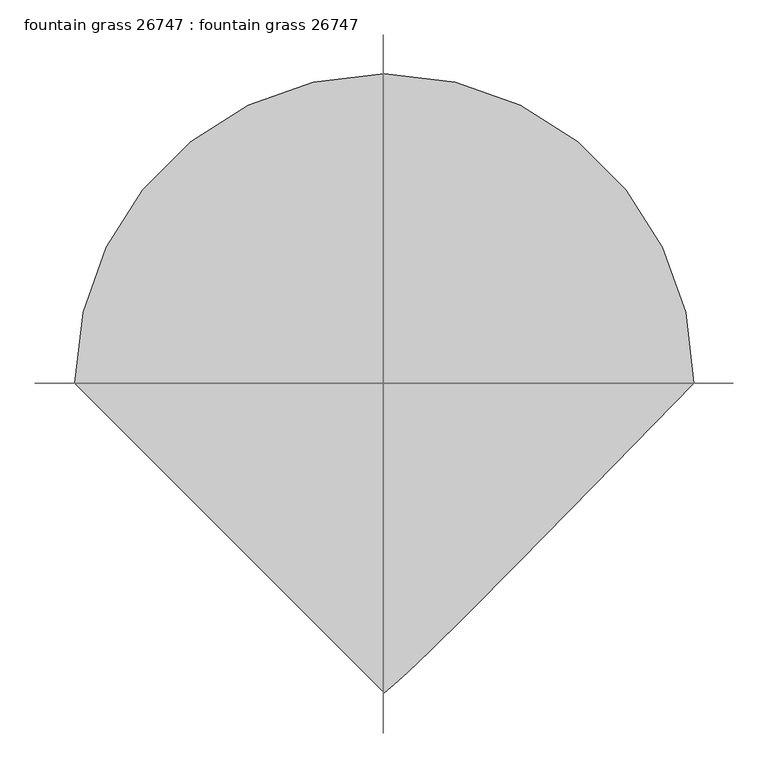
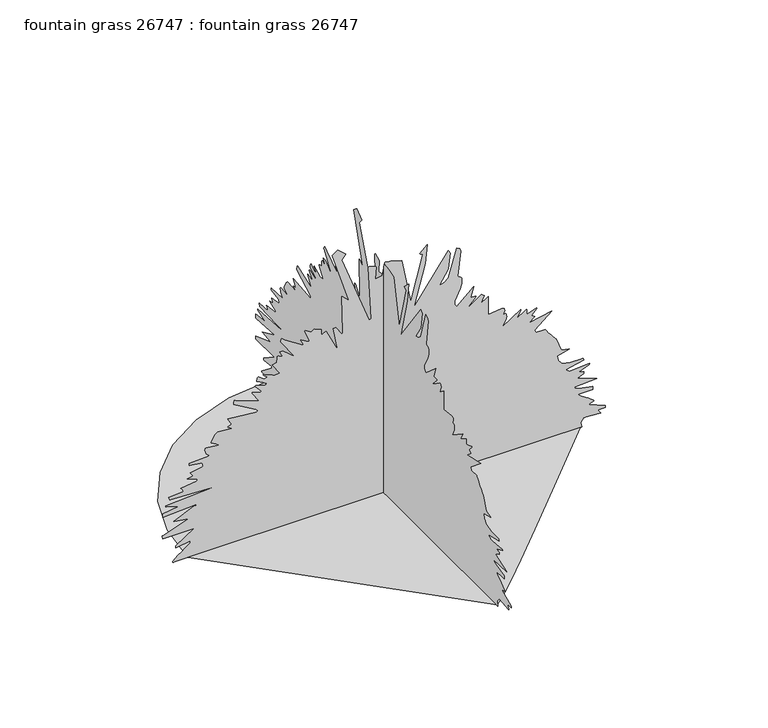
"""IFC4 building model written with IfcOpenShell, lengths in millimetres: proxy geometry, fountain grass 26747 : fountain grass 26747."""

from ifc_helpers import new_model, si_unit, origin, place, context, project, spatial, triangles, source, transform, mapped, element, save


def fountain_grass_26747_fountain_grass_26747_29f4d5b1(model_context):
    return source(origin(), model_context, "Body", "Tessellation", [
        triangles([(-987.0455658, 0.0, 0.0001807), (-960.952173, 226.1654466, 0.0001807), (-886.6343983, 433.862035, 0.0001807), (-770.0484913, 617.1406734, 0.0001807), (-617.1406734, 770.0484913, 0.0001807), (-433.862035, 886.6343983, 0.0001807), (-226.1654466, 960.952173, 0.0001807), (4.31e-05, 987.0455658, 0.0001807), (226.1657009, 960.952173, 0.0001807), (433.862035, 886.6343983, 0.0001807), (617.1406734, 770.0484913, 0.0001807), (770.0484913, 617.1406734, 0.0001807), (886.6343983, 433.862035, 0.0001807), (960.952173, 226.1654466, 0.0001807), (987.0455658, -8.63e-05, 0.0001807), (666.2769184, -329.0287173, 0.0001807), (428.4772619, -571.2784656, 0.0001807), (259.8137924, -741.2118793, 0.0001807), (146.4631077, -853.2918114, 0.0001807), (74.5956602, -921.9810053, 0.0001807), (30.3837036, -961.7446392, 0.0001807), (-0.0001294, -987.0455658, 0.0001807), (-192.732222, 8.8e-06, 1335.7745705), (-213.2038286, 7.2e-06, 1310.1839813), (-75.0206025, -1.47e-05, 941.6939009), (-74.0421966, -1.47e-05, 941.9784039), (-72.5994794, -1.47e-05, 942.7098999), (-70.8743122, -1.46e-05, 943.7080948), (-69.0480519, -1.45e-05, 944.7977812), (-67.3038361, -1.45e-05, 945.7985195), (-65.8220043, -1.44e-05, 946.5300882), (-64.7846675, -1.44e-05, 946.8119751), (-80.1384406, 2.1e-06, 1223.1789722), (-79.3512975, 2.1e-06, 1223.3695129), (-78.4244554, 2.1e-06, 1223.8850338), (-77.4526488, 2.1e-06, 1224.6394936), (-76.5311389, 2.2e-06, 1225.5436535), (-75.2199908, 2.3e-06, 1227.4587982), (-75.0206025, 2.4e-06, 1228.2971191), (-39.1952093, 1.4e-06, 1212.9427511), (-44.3130519, -2.2e-06, 1151.5281858), (-8.4877319, -1.9e-06, 1156.6462601), (4.7327266, 1.8e-06, 1221.0427654), (6.8660195, 2.1e-06, 1223.1789722), (43.5436857, 1.6e-06, 1215.9958351), (88.7523407, 8e-07, 1202.7066027), (134.8136643, -1.32e-05, 967.2843447), (196.2285203, 5e-07, 1197.5909992), (183.550624, 1e-06, 1203.2526449), (181.3428736, 1.1e-06, 1205.4269308), (180.8747518, 1.1e-06, 1207.8246769), (216.700145, 3.3e-06, 1243.6512691), (206.4644507, -2.5e-06, 1146.4100389), (150.1674419, -1.53e-05, 931.4576797), (324.1773419, 3.2e-06, 1172.2011972), (334.4109833, 2.3e-06, 1156.8469019), (324.1773419, -2.6e-06, 1074.959967), (278.1144741, -6.8e-06, 1003.3091806), (303.186799, -6.4e-06, 1010.2737991), (322.3333048, -5.3e-06, 1028.8183794), (365.1195376, 3.2e-06, 1172.2011972), (380.7405318, 2.8e-06, 1165.3635332), (386.8136713, 1.8e-06, 1149.1050053), (371.0377447, -5.8e-06, 1020.4236883), (372.5033166, -6e-06, 1017.0835579), (375.3150999, -6.2e-06, 1014.6375589), (378.9295232, -6.3e-06, 1012.7299719), (382.8157322, -6.4e-06, 1011.0028244), (386.4301191, -6.5e-06, 1009.0952374), (389.2419024, -6.6e-06, 1006.6492384), (390.7100178, -6.8e-06, 1003.3091806), (390.8116467, -8.5e-06, 974.9780611), (383.7479064, -1e-05, 950.4898756), (355.0433722, -1.34e-05, 892.7557543), (354.7944775, -1.44e-05, 876.299128), (365.1195376, -1.54e-05, 860.0101513), (452.1246194, -1.08e-05, 936.7764685), (436.7703604, -1.39e-05, 885.5980516), (437.4358357, -1.38e-05, 884.2035873), (460.8495229, -1.41e-05, 882.1284233), (462.3608042, -1.42e-05, 880.4799774), (460.8800079, -1.46e-05, 876.8274387), (425.4318083, -1.61e-05, 841.6561117), (426.5341393, -1.66e-05, 839.537709), (430.7911832, -1.6e-05, 840.3353348), (487.9487409, -1.42e-05, 880.4799774), (489.1120783, -1.43e-05, 881.361319), (491.0831062, -1.43e-05, 880.6425402), (503.3030362, -1.48e-05, 870.2437563), (487.9487409, -1.69e-05, 834.4196348), (523.7754058, -1.54e-05, 860.0101513), (523.7754058, -2.12e-05, 762.7688484), (593.7116893, -2.08e-05, 769.8782982), (604.2222033, -2.1e-05, 765.8219324), (607.2778307, -2.16e-05, 755.5679798), (600.5443027, -2.27e-05, 737.1784046), (610.7779804, -2.27e-05, 737.1784046), (611.8422323, -2.27e-05, 736.5230667), (614.1129513, -2.29e-05, 734.0897123), (616.2186367, -2.32e-05, 729.1722799), (616.7773962, -2.37e-05, 721.0722656), (614.4152584, -2.44e-05, 709.086006), (595.4261922, -2.67e-05, 670.6456924), (687.546841, -2.3e-05, 732.0602577), (687.8186268, -2.35e-05, 728.1842588), (667.0770149, -2.55e-05, 691.118062), (716.0887762, -2.38e-05, 722.0933516), (718.2554317, -2.36e-05, 721.8266527), (719.3450455, -2.39e-05, 719.0986942), (717.5061316, -2.5e-05, 697.6534916), (718.2554317, -2.51e-05, 696.2361362), (720.4347319, -2.49e-05, 695.6976517), (766.5382404, -2.45e-05, 712.7029364), (769.4337759, -2.42e-05, 711.5904316), (768.6387663, -2.44e-05, 709.4415802), (744.2522461, -2.59e-05, 683.2440514), (743.8433321, -2.61e-05, 680.8819136), (759.1976274, -2.67e-05, 670.6456924), (728.4915802, -2.82e-05, 645.0577194), (845.0825741, -2.67e-05, 669.6881201), (759.1976274, -3.09e-05, 598.994906), (764.3157017, -3.19e-05, 583.6431541), (810.3760443, -3.19e-05, 583.6431541), (812.6900019, -3.21e-05, 579.4623047), (818.8519804, -3.26e-05, 570.8923699), (827.7013676, -3.33e-05, 559.353176), (838.0696301, -3.41e-05, 546.269636), (848.7985537, -3.49e-05, 533.064192), (858.7223665, -3.56e-05, 521.1643006), (866.6750788, -3.61e-05, 511.9923677), (892.2629791, -4.01e-05, 445.4596919), (933.2077909, -4.07e-05, 435.2234708), (871.793153, -4.16e-05, 419.8692118), (876.9112272, -4.31e-05, 394.2787316), (879.8754358, -4.33e-05, 391.6269676), (882.8904408, -4.35e-05, 388.2919604), (885.7733316, -4.37e-05, 384.6267408), (888.3361839, -4.39e-05, 380.9920063), (890.3960873, -4.41e-05, 377.7407876), (891.7651897, -4.43e-05, 375.2261882), (892.2629791, -4.44e-05, 373.8088692), (895.890156, -4.44e-05, 372.7801892), (938.3258652, -4.5e-05, 363.5726844), (999.7404305, -4.5e-05, 363.5726844), (1000.5278824, -4.5e-05, 362.5440044), (1001.4549334, -4.51e-05, 361.080976), (1002.425223, -4.52e-05, 359.3588428), (1003.3472597, -4.53e-05, 357.5503776), (1004.1219217, -4.54e-05, 355.8282443), (1004.6578629, -4.55e-05, 354.3652159), (1004.8585773, -4.56e-05, 353.3364996), (912.7354214, -4.68e-05, 332.86413), (913.6015022, -4.69e-05, 331.6373154), (915.8976557, -4.7e-05, 329.6383458), (919.1819029, -4.71e-05, 327.1415142), (923.0020912, -4.73e-05, 324.4110123), (926.9110823, -4.75e-05, 321.7160823), (930.4620283, -4.76e-05, 319.3259302), (933.2077909, -4.77e-05, 317.5123781), (949.6695042, -4.77e-05, 318.6757155), (1032.0797356, -4.76e-05, 324.6954789), (1035.5645519, -4.74e-05, 322.6279452), (1033.032221, -4.76e-05, 319.7526484), (979.2680609, -4.89e-05, 297.0400085), (1004.8585773, -4.92e-05, 291.9219162), (1004.8585773, -4.99e-05, 281.6857132), (975.3971489, -5.07e-05, 267.6446189), (974.1499866, -5.08e-05, 266.331436), (1071.3912169, -5.29e-05, 230.5068058), (958.7956913, -5.32e-05, 225.3889678), (958.7956913, -5.35e-05, 220.2708572), (979.2680609, -5.41e-05, 210.0351811), (1050.9188473, -5.5e-05, 194.6814126), (1050.9188473, -5.6e-05, 179.327626), (974.1499866, -5.6e-05, 179.327626), (978.767728, -5.62e-05, 175.5818881), (990.6523224, -5.67e-05, 167.0838239), (1006.8625975, -5.74e-05, 155.6789786), (1024.4520761, -5.81e-05, 143.2134423), (1051.9830992, -5.94e-05, 122.4842661), (1056.0369942, -5.96e-05, 117.9127791), (1055.1428627, -5.97e-05, 116.2480642), (1031.9527084, -6.02e-05, 108.5996212), (1030.4464777, -6.02e-05, 107.6770939), (1112.3334852, -6.24e-05, 71.8517007), (1112.3334852, -6.3e-05, 61.6157658), (1076.5093637, -6.3e-05, 61.6157658), (1088.8461107, -6.4e-05, 43.7974311), (1091.8611156, -6.42e-05, 41.1441501), (1004.8585773, -6.39e-05, 46.2622425), (989.504282, -6.51e-05, 25.7906269), (994.6223562, -6.66e-05, 0.2009925), (-1062.775609, -7.09e-05, 6.89e-05), (-1062.775609, -7.05e-05, 5.1179681), (-1049.4888474, -6.99e-05, 15.7529118), (-1033.944084, -6.92e-05, 27.9602914), (-1017.6728388, -6.84e-05, 40.5703616), (-1002.191589, -6.77e-05, 52.4138656), (-989.0343979, -6.71e-05, 62.3213777), (-979.7176701, -6.67e-05, 69.1234924), (-975.7730707, -6.66e-05, 71.6507864), (-975.7730707, -6.6e-05, 81.8864716), (-1047.4213137, -6.66e-05, 71.6507864), (-1047.4213137, -6.6e-05, 81.8864716), (-955.3006285, -6.23e-05, 143.3013185), (-1113.9564966, -6.23e-05, 143.3013185), (-1114.0479881, -6.22e-05, 144.6553964), (-1114.2638906, -6.21e-05, 147.0447673), (-1114.5102419, -6.19e-05, 150.0158069), (-1114.6931522, -6.17e-05, 153.1156177), (-1114.7261444, -6.16e-05, 155.891066), (-1114.5102419, -6.14e-05, 157.8885276), (-1113.9564966, -6.14e-05, 158.6551051), (-986.0066757, -5.87e-05, 204.7161744), (-1054.7643974, -5.81e-05, 213.3275311), (-1057.6574621, -5.8e-05, 214.9521049), (-955.3006285, -5.53e-05, 261.0126836), (-945.06448, -5.53e-05, 261.0126836), (-945.06448, -5.5e-05, 266.130776), (-1113.9564966, -5.56e-05, 255.8945912), (-1113.9564966, -5.44e-05, 276.3669608), (-1032.0695618, -5.38e-05, 286.6031456), (-1098.6022739, -5.26e-05, 307.0755152), (-1098.6022739, -5.22e-05, 312.1910823), (-852.941324, -5.13e-05, 327.5453776), (-1078.1298317, -5.07e-05, 337.7815624), (-1082.9660191, -4.99e-05, 351.3121319), (-1083.2479786, -4.98e-05, 353.1358578), (-1006.4790453, -4.95e-05, 358.253932), (-1021.1679016, -4.84e-05, 377.3064754), (-1021.8333406, -4.83e-05, 378.7237945), (-939.9464058, -4.77e-05, 388.9599792), (-939.9464058, -4.71e-05, 399.196164), (-983.6648129, -4.62e-05, 414.4208888), (-989.0952953, -4.6e-05, 417.5603411), (-991.1248226, -4.58e-05, 419.6685336), (-960.4187754, -4.55e-05, 424.7866442), (-975.1050156, -4.44e-05, 443.8391513), (-975.7730707, -4.43e-05, 445.2590137), (-909.2403585, -4.37e-05, 455.4926551), (-914.3558893, -4.25e-05, 475.965061), (-980.8911449, -4.19e-05, 486.2012458), (-980.8911449, -4.13e-05, 496.4374306), (-878.5317678, -4.1e-05, 501.5555048), (-879.1134184, -4.09e-05, 503.3716003), (-888.6028828, -4.02e-05, 513.6840159), (-893.8860632, -4e-05, 516.9098001), (-900.7211838, -3.88e-05, 540.5851356), (-900.558621, -3.85e-05, 544.4840255), (-899.0041374, -3.82e-05, 547.6158474), (-894.7090508, -3.84e-05, 548.9721963), (-839.7257063, -3.85e-05, 543.0539892), (-832.4714979, -3.85e-05, 542.4977368), (-834.0945093, -3.85e-05, 545.8555987), (-865.9461262, -3.72e-05, 565.5888419), (-868.2956194, -3.7e-05, 568.088217), (-868.4048424, -3.65e-05, 572.164894), (-848.5039495, -3.46e-05, 604.96896), (-842.4562082, -3.44e-05, 611.1792641), (-837.5895721, -3.42e-05, 614.1485596), (-765.9387857, -3.46e-05, 609.030449), (-780.5183464, -3.41e-05, 617.4352776), (-785.6364206, -3.37e-05, 622.5609821), (-786.4086119, -3.36e-05, 624.384708), (-767.3586119, -3.34e-05, 628.6646067), (-765.9387857, -3.33e-05, 629.5027822), (-786.4086119, -3.12e-05, 665.3269037), (-637.9889648, -3.21e-05, 649.9752245), (-637.7984241, -3.21e-05, 650.9530718), (-637.2828306, -3.2e-05, 652.395789), (-636.5284435, -3.19e-05, 654.1204657), (-635.6242109, -3.18e-05, 655.946735), (-634.6564648, -3.17e-05, 657.6916866), (-633.7090662, -3.16e-05, 659.1725555), (-632.8733614, -3.15e-05, 660.2088295), (-755.7025646, -2.72e-05, 731.8596159), (-755.710195, -2.71e-05, 734.6180958), (-755.6593987, -2.69e-05, 738.1944036), (-755.4384092, -2.67e-05, 742.1339161), (-754.9329895, -2.65e-05, 745.9743793), (-754.0313004, -2.63e-05, 749.26117), (-752.6190319, -2.61e-05, 751.5344324), (-750.5844904, -2.6e-05, 752.3319855), (-627.7552872, -2.88e-05, 706.2717155), (-663.6860882, -2.56e-05, 759.6675116), (-663.5794086, -2.54e-05, 762.5682066), (-660.4755283, -2.56e-05, 763.5054314), (-620.4934484, -2.58e-05, 751.3083561), (-617.5191387, -2.6e-05, 752.3319855), (-618.27854, -2.56e-05, 755.4434961), (-647.6638103, -2.37e-05, 790.1982788), (-648.2251133, -2.36e-05, 793.2742538), (-645.0653498, -2.38e-05, 794.1149729), (-597.0467328, -2.45e-05, 777.9225019), (-596.4675894, -2.44e-05, 778.9130665), (-595.0452198, -2.43e-05, 780.3888485), (-593.2570295, -2.42e-05, 782.1490608), (-591.5755551, -2.41e-05, 784.0032354), (-590.4782747, -2.4e-05, 785.7507305), (-590.4376522, -2.39e-05, 787.201078), (-591.9286222, -2.39e-05, 788.1586504), (-637.9889648, -2.24e-05, 813.7466234), (-639.6145197, -2.21e-05, 815.2045286), (-640.0666723, -2.19e-05, 818.265243), (-638.3851616, -2.15e-05, 826.5253492), (-636.7163681, -2.14e-05, 830.3861601), (-634.8012234, -2.12e-05, 833.1724726), (-632.8733614, -2.11e-05, 834.218993), (-630.4730719, -2.12e-05, 834.2443548), (-602.164807, -2.24e-05, 813.7466234), (-586.810548, -2.2e-05, 818.8646976), (-606.0256179, -2.11e-05, 834.9200403), (-607.7909171, -2.1e-05, 837.6987951), (-607.2829176, -2.08e-05, 839.3370672), (-603.6684943, -2.09e-05, 838.9128925), (-561.8702826, -2.2e-05, 820.0915123), (-550.9864265, -2.24e-05, 813.7466234), (-525.3959464, -2.2e-05, 818.8646976), (-559.8662261, -1.89e-05, 871.7906096), (-561.2226113, -1.87e-05, 875.1611887), (-540.7502054, -1.84e-05, 880.2793356), (-537.9714506, -1.73e-05, 906.7536644), (-536.9859366, -1.7e-05, 909.870262), (-535.6321312, -1.66e-05, 910.9878536), (-533.2191244, -1.68e-05, 912.2654646), (-529.3558064, -1.69e-05, 911.5212513), (-510.0416511, -1.72e-05, 900.7517052), (-525.3959464, -1.53e-05, 931.4576797), (-510.0416511, -1.53e-05, 931.4576797), (-448.6270494, -1.84e-05, 880.2793356), (-520.2778358, -1.23e-05, 982.63864), (-520.4962818, -1.22e-05, 984.7163475), (-516.051277, -1.16e-05, 996.9642191), (-515.2257823, -1.15e-05, 998.3459661), (-515.1597616, -1.14e-05, 997.9903919), (-498.3728866, -1.21e-05, 985.7882298), (-408.0734565, -1.55e-05, 927.9093498), (-402.5667432, -1.56e-05, 926.342149), (-417.4790597, -1.45e-05, 951.9148613), (-418.5687098, -1.42e-05, 955.282897), (-417.9210385, -1.38e-05, 957.0481962), (-415.5080317, -1.41e-05, 957.1853245), (-380.6389392, -1.48e-05, 937.1701944), (-376.976263, -1.5e-05, 936.5758266), (-376.9203798, -1.43e-05, 940.7439589), (-397.9032924, -1.21e-05, 994.048336), (-397.4486326, -1.14e-05, 997.9903919), (-395.0686543, -1.16e-05, 998.5085289), (-366.1584277, -1.23e-05, 982.382115), (-351.3883264, -1.17e-05, 992.8748611), (-315.5616614, -1.26e-05, 977.5205658), (-315.5616614, -1.44e-05, 946.8119751), (-294.1621864, -1.4e-05, 958.3587994), (-291.1294318, -1.39e-05, 958.6407589), (-289.9737247, -1.38e-05, 957.0481962), (-233.6754533, -2.08e-05, 839.3370672), (-254.1470598, -1.35e-05, 962.1662704), (-243.9113837, -1.35e-05, 962.1662704), (-213.2038286, -1.62e-05, 916.1059278), (-211.0877513, -1.6e-05, 916.598703), (-209.5368286, -1.59e-05, 917.6680418), (-208.4642015, -1.57e-05, 919.1971636), (-207.7817031, -1.56e-05, 921.0716858), (-207.4032379, -1.54e-05, 923.1722116), (-207.2399121, -1.53e-05, 925.3845766), (-207.2046126, -1.52e-05, 927.5918547), (-213.2038286, -4.4e-06, 1115.7040644), (-210.5383663, -4.8e-06, 1115.4424524), (-179.2496511, -6.1e-06, 1087.4745375), (-177.3786897, -6.2e-06, 1084.9954737), (-259.2651522, 9.7e-06, 1351.1262497), (-233.6754533, 1.09e-05, 1371.5986919), (-3.3699163, 189.3624059, 1335.7745705), (-3.3699163, 209.8340125, 1310.1839813), (-3.3699163, 71.6505366, 941.6939009), (-3.3699163, 70.6721261, 941.9784039), (-3.3699163, 69.2296633, 942.7098999), (-3.3699163, 67.5042417, 943.7080948), (-3.3699163, 65.6782403, 944.7977812), (-3.3699163, 63.93402, 945.7985195), (-3.3699163, 62.4519338, 946.5300882), (-3.3699163, 61.4148514, 946.8119751), (-3.3699163, 76.7683792, 1223.1789722), (-3.3699163, 75.9812316, 1223.3695129), (-3.3699163, 75.054385, 1223.8850338), (-3.3699163, 74.0828373, 1224.6394936), (-3.3699163, 73.161073, 1225.5436535), (-3.3699163, 71.8499249, 1227.4587982), (-3.3699163, 71.6505366, 1228.2971191), (-3.3699163, 35.8251411, 1212.9427511), (-3.3699163, 40.9429814, 1151.5281858), (-3.3699163, 5.1177648, 1156.6462601), (-3.3699163, -8.1026934, 1221.0427654), (-3.3699163, -10.2359611, 1223.1789722), (-3.3699163, -46.9137516, 1215.9958351), (-3.3699163, -92.122402, 1202.7066027), (-3.3699163, -138.1834804, 967.2843447), (-3.3699163, -199.5985907, 1197.5909992), (-3.3699163, -186.9206945, 1203.2526449), (-3.3699163, -184.7129259, 1205.4269308), (-3.3699163, -184.244804, 1207.8246769), (-3.3699163, -220.0701972, 1243.6512691), (-3.3699163, -209.8342668, 1146.4100389), (-3.3699163, -153.5372671, 931.4576797), (-3.3699163, -327.5453776, 1172.2011972), (-3.3699163, -337.7815624, 1156.8469019), (-3.3699163, -327.5453776, 1074.959967), (-3.3699163, -281.4850532, 1003.3091806), (-3.3699163, -306.5573782, 1010.2737991), (-3.3699163, -325.7038839, 1028.8183794), (-3.3699163, -368.4901168, 1172.2011972), (-3.3699163, -384.1085675, 1165.3635332), (-3.3699163, -390.1842505, 1149.1050053), (-3.3699163, -374.4057804, 1020.4236883), (-3.3699163, -375.8738957, 1017.0835579), (-3.3699163, -378.6856791, 1014.6375589), (-3.3699163, -382.3001023, 1012.7299719), (-3.3699163, -386.1863113, 1011.0028244), (-3.3699163, -389.8006983, 1009.0952374), (-3.3699163, -392.6124816, 1006.6492384), (-3.3699163, -394.0780535, 1003.3091806), (-3.3699163, -394.1796824, 974.9780611), (-3.3699163, -387.1184855, 950.4898756), (-3.3699163, -358.4139513, 892.7557543), (-3.3699163, -358.1650566, 876.299128), (-3.3699163, -368.4901168, 860.0101513), (-3.3699163, -455.4926551, 936.7764685), (-3.3699163, -440.1409032, 885.5980516), (-3.3699163, -440.8038714, 884.2035873), (-3.3699163, -464.2175586, 882.1284233), (-3.3699163, -465.7288399, 880.4799774), (-3.3699163, -464.2505871, 876.8274387), (-3.3699163, -428.8023874, 841.6561117), (-3.3699163, -429.9047184, 839.537709), (-3.3699163, -434.1617623, 840.3353348), (-3.3699163, -491.31932, 880.4799774), (-3.3699163, -492.480114, 881.361319), (-3.3699163, -494.4536854, 880.6425402), (-3.3699163, -506.6736154, 870.2437563), (-3.3699163, -491.31932, 834.4196348), (-3.3699163, -527.1434415, 860.0101513), (-3.3699163, -527.1434415, 762.7688484), (-3.3699163, -597.079725, 769.8782982), (-3.3699163, -607.5927824, 765.8219324), (-3.3699163, -610.6458664, 755.5679798), (-3.3699163, -603.9123384, 737.1784046), (-3.3699163, -614.1485596, 737.1784046), (-3.3699163, -615.2128115, 736.5230667), (-3.3699163, -617.4835304, 734.0897123), (-3.3699163, -619.5866724, 729.1722799), (-3.3699163, -620.1479753, 721.0722656), (-3.3699163, -617.7858376, 709.086006), (-3.3699163, -598.7942279, 670.6456924), (-3.3699163, -690.9174202, 732.0602577), (-3.3699163, -691.1866625, 728.1842588), (-3.3699163, -670.4450506, 691.118062), (-3.3699163, -719.4568119, 722.0933516), (-3.3699163, -721.6260109, 721.8266527), (-3.3699163, -722.7156246, 719.0986942), (-3.3699163, -720.8767107, 697.6534916), (-3.3699163, -721.6260109, 696.2361362), (-3.3699163, -723.805311, 695.6976517), (-3.3699163, -769.9062761, 712.7029364), (-3.3699163, -772.804355, 711.5904316), (-3.3699163, -772.0093454, 709.4415802), (-3.3699163, -747.6202818, 683.2440514), (-3.3699163, -747.2139112, 680.8819136), (-3.3699163, -762.5682066, 670.6456924), (-3.3699163, -731.8596159, 645.0577194), (-3.3699163, -848.4531532, 669.6881201), (-3.3699163, -762.5682066, 598.994906), (-3.3699163, -767.6862808, 583.6431541), (-3.3699163, -813.7466234, 583.6431541), (-3.3699163, -816.0605083, 579.4623047), (-3.3699163, -822.2225595, 570.8923699), (-3.3699163, -831.0694033, 559.353176), (-3.3699163, -841.4402092, 546.269636), (-3.3699163, -852.1691328, 533.064192), (-3.3699163, -862.0904022, 521.1643006), (-3.3699163, -870.0431145, 511.9923677), (-3.3699163, -895.6335583, 445.4596919), (-3.3699163, -936.5758266, 435.2234708), (-3.3699163, -875.1611887, 419.8692118), (-3.3699163, -880.2793356, 394.2787316), (-3.3699163, -883.246015, 391.6269676), (-3.3699163, -886.2610199, 388.289417), (-3.3699163, -889.1439108, 384.6267408), (-3.3699163, -891.7067631, 380.9920063), (-3.3699163, -893.764123, 377.7407876), (-3.3699163, -895.1357689, 375.2261882), (-3.3699163, -895.6335583, 373.8088692), (-3.3699163, -899.2607351, 372.7801892), (-3.3699163, -941.6939009, 363.5726844), (-3.3699163, -1003.1084661, 363.5726844), (-3.3699163, -1003.8959181, 362.5440044), (-3.3699163, -1004.8229691, 361.080976), (-3.3699163, -1005.7958021, 359.3588428), (-3.3699163, -1006.7178389, 357.5503776), (-3.3699163, -1007.4925009, 355.8282443), (-3.3699163, -1008.028442, 354.3652159), (-3.3699163, -1008.226613, 353.3364996), (-3.3699163, -916.1059278, 332.86413), (-3.3699163, -916.9695379, 331.6373154), (-3.3699163, -919.2682348, 329.6383458), (-3.3699163, -922.5499386, 327.1415142), (-3.3699163, -926.3701269, 324.4110123), (-3.3699163, -930.279118, 321.7160823), (-3.3699163, -933.8326075, 319.3259302), (-3.3699163, -936.5758266, 317.5098347), (-3.3699163, -953.0400833, 318.6757155), (-3.3699163, -1035.4503147, 324.6954789), (-3.3699163, -1038.9351311, 322.6279452), (-3.3699163, -1036.4028002, 319.7501049), (-3.3699163, -982.63864, 297.0400085), (-3.3699163, -1008.226613, 291.9219162), (-3.3699163, -1008.226613, 281.6857132), (-3.3699163, -978.767728, 267.6446189), (-3.3699163, -977.5205658, 266.331436), (-3.3699163, -1074.7592525, 230.5068058), (-3.3699163, -962.1662704, 225.3887135), (-3.3699163, -962.1662704, 220.2708572), (-3.3699163, -982.63864, 210.0351811), (-3.3699163, -1054.2894264, 194.6814126), (-3.3699163, -1054.2894264, 179.327626), (-3.3699163, -977.5205658, 179.327626), (-3.3699163, -982.1357637, 175.5818881), (-3.3699163, -994.0229015, 167.0835696), (-3.3699163, -1010.2331766, 155.6787243), (-3.3699163, -1027.8226553, 143.2131879), (-3.3699163, -1055.3536783, 122.4842661), (-3.3699163, -1059.4075733, 117.9127791), (-3.3699163, -1058.5134418, 116.2478099), (-3.3699163, -1035.3207441, 108.5993669), (-3.3699163, -1033.8170568, 107.6768396), (-3.3699163, -1115.7040644, 71.8517007), (-3.3699163, -1115.7040644, 61.6157658), (-3.3699163, -1079.8773994, 61.6157658), (-3.3699163, -1092.2166899, 43.7971768), (-3.3699163, -1095.2316948, 41.1441501), (-3.3699163, -1008.226613, 46.2619882), (-3.3699163, -992.8748611, 25.7903726), (-3.3699163, -997.9929354, 0.2009237), (-3.3699163, 1059.4050299, 0.0), (-3.3699163, 1059.4050299, 5.117917), (-3.3699163, 1046.1182682, 15.7528607), (-3.3699163, 1030.5760483, 27.9600371), (-3.3699163, 1014.3022596, 40.5701072), (-3.3699163, 998.8235533, 52.4138656), (-3.3699163, 985.6638187, 62.3213777), (-3.3699163, 976.3496344, 69.1234924), (-3.3699163, 972.4024916, 71.6507864), (-3.3699163, 972.4024916, 81.8864716), (-3.3699163, 1044.053278, 71.6507864), (-3.3699163, 1044.053278, 81.8864716), (-3.3699163, 951.930122, 143.3013185), (-3.3699163, 1110.5859175, 143.3013185), (-3.3699163, 1110.677409, 144.6553964), (-3.3699163, 1110.8933115, 147.0447673), (-3.3699163, 1111.1396627, 150.0158069), (-3.3699163, 1111.3251165, 153.1156177), (-3.3699163, 1111.3555653, 155.891066), (-3.3699163, 1111.1396627, 157.8885276), (-3.3699163, 1110.5859175, 158.6551051), (-3.3699163, 982.63864, 204.7161744), (-3.3699163, 1051.3938183, 213.3275311), (-3.3699163, 1054.2894264, 214.9521049), (-3.3699163, 951.930122, 261.0126836), (-3.3699163, 941.6939009, 261.0126836), (-3.3699163, 941.6939009, 266.130776), (-3.3699163, 1110.5859175, 255.8945912), (-3.3699163, 1110.5859175, 276.3669608), (-3.3699163, 1028.6989826, 286.6031456), (-3.3699163, 1095.2316948, 307.0755152), (-3.3699163, 1095.2316948, 312.1910823), (-3.3699163, 849.5732883, 327.5453776), (-3.3699163, 1074.7592525, 337.7815624), (-3.3699163, 1079.5954399, 351.3121319), (-3.3699163, 1079.8773994, 353.1358578), (-3.3699163, 1003.1084661, 358.253932), (-3.3699163, 1017.7973225, 377.3064754), (-3.3699163, 1018.4627615, 378.7237945), (-3.3699163, 936.5758266, 388.9599792), (-3.3699163, 936.5758266, 399.196164), (-3.3699163, 980.2942337, 414.4208888), (-3.3699163, 985.7272596, 417.5603411), (-3.3699163, 987.7567869, 419.6685336), (-3.3699163, 957.0481962, 424.7866442), (-3.3699163, 971.7369799, 443.8391513), (-3.3699163, 972.4024916, 445.2590137), (-3.3699163, 905.8697794, 455.4926551), (-3.3699163, 910.9878536, 475.965061), (-3.3699163, 977.5205658, 486.2012458), (-3.3699163, 977.5205658, 496.4374306), (-3.3699163, 875.1611887, 501.5555048), (-3.3699163, 875.7428392, 503.3690932), (-3.3699163, 885.2348471, 513.6814725), (-3.3699163, 890.515484, 516.9098001), (-3.3699163, 897.3506046, 540.5851356), (-3.3699163, 897.1880419, 544.4840255), (-3.3699163, 895.6335583, 547.6158474), (-3.3699163, 891.3384716, 548.9721963), (-3.3699163, 836.3576706, 543.0539892), (-3.3699163, 829.1009188, 542.4977368), (-3.3699163, 830.7239302, 545.8555987), (-3.3699163, 862.5780905, 565.5888419), (-3.3699163, 864.9250402, 568.088217), (-3.3699163, 865.0368067, 572.1623506), (-3.3699163, 845.1333704, 604.96896), (-3.3699163, 839.0856291, 611.1792641), (-3.3699163, 834.218993, 614.1485596), (-3.3699163, 762.5682066, 609.030449), (-3.3699163, 777.1477673, 617.4352776), (-3.3699163, 782.2658415, 622.5609821), (-3.3699163, 783.0405762, 624.384708), (-3.3699163, 763.9880327, 628.6646067), (-3.3699163, 762.5682066, 629.5027822), (-3.3699163, 783.0405762, 665.3269037), (-3.3699163, 634.6209291, 649.9752245), (-3.3699163, 634.427845, 650.9530718), (-3.3699163, 633.9122515, 652.395789), (-3.3699163, 633.1604078, 654.1204657), (-3.3699163, 632.2561752, 655.946735), (-3.3699163, 631.2858856, 657.6916866), (-3.3699163, 630.3410305, 659.1725555), (-3.3699163, 629.5027822, 660.2088295), (-3.3699163, 752.3319855, 731.8596159), (-3.3699163, 752.3396158, 734.6180958), (-3.3699163, 752.291363, 738.1944036), (-3.3699163, 752.0703735, 742.1339161), (-3.3699163, 751.5649538, 745.9743793), (-3.3699163, 750.6632647, 749.26117), (-3.3699163, 749.2484528, 751.5344324), (-3.3699163, 747.2139112, 752.3319855), (-3.3699163, 624.384708, 706.2717155), (-3.3699163, 660.315509, 759.6675116), (-3.3699163, 660.2088295, 762.5682066), (-3.3699163, 657.1049492, 763.5054314), (-3.3699163, 617.1228693, 751.3083561), (-3.3699163, 614.1485596, 752.3319855), (-3.3699163, 614.9079609, 755.4434961), (-3.3699163, 644.2932312, 790.1982788), (-3.3699163, 644.8570776, 793.2742538), (-3.3699163, 641.6947706, 794.1149729), (-3.3699163, 593.6761537, 777.9225019), (-3.3699163, 593.0970102, 778.9130665), (-3.3699163, 591.6771841, 780.3888485), (-3.3699163, 589.8864867, 782.1490608), (-3.3699163, 588.2075194, 784.0032354), (-3.3699163, 587.1076956, 785.7507305), (-3.3699163, 587.0670731, 787.201078), (-3.3699163, 588.5580431, 788.1586504), (-3.3699163, 634.6209291, 813.7466234), (-3.3699163, 636.2439405, 815.2045286), (-3.3699163, 636.6960932, 818.265243), (-3.3699163, 635.0171259, 826.5253492), (-3.3699163, 633.3458616, 830.3861601), (-3.3699163, 631.4306442, 833.1724726), (-3.3699163, 629.5027822, 834.218993), (-3.3699163, 627.1050362, 834.2443548), (-3.3699163, 598.7942279, 813.7466234), (-3.3699163, 583.4399689, 818.8646976), (-3.3699163, 602.6575822, 834.9200403), (-3.3699163, 604.420338, 837.6987951), (-3.3699163, 603.9123384, 839.3370672), (-3.3699163, 600.2979152, 838.9128925), (-3.3699163, 558.5022469, 820.0915123), (-3.3699163, 547.6158474, 813.7466234), (-3.3699163, 522.0253673, 818.8646976), (-3.3699163, 556.495647, 871.7906096), (-3.3699163, 557.8520322, 875.1611887), (-3.3699163, 537.3796263, 880.2793356), (-3.3699163, 534.6008715, 906.7536644), (-3.3699163, 533.6153575, 909.870262), (-3.3699163, 532.261552, 910.9878536), (-3.3699163, 529.8510887, 912.2654646), (-3.3699163, 525.9877707, 911.5212513), (-3.3699163, 506.6736154, 900.7517052), (-3.3699163, 522.0253673, 931.4576797), (-3.3699163, 506.6736154, 931.4576797), (-3.3699163, 445.2564703, 880.2793356), (-3.3699163, 516.9072567, 982.63864), (-3.3699163, 517.1282461, 984.7163475), (-3.3699163, 512.6832413, 996.9642191), (-3.3699163, 511.8552032, 998.3459661), (-3.3699163, 511.7891825, 997.9929354), (-3.3699163, 495.0023074, 985.7882298), (-3.3699163, 404.7028773, 927.9093498), (-3.3699163, 399.196164, 926.342149), (-3.3699163, 414.111024, 951.9148613), (-3.3699163, 415.1981306, 955.282897), (-3.3699163, 414.5504594, 957.0481962), (-3.3699163, 412.1374526, 957.1853245), (-3.3699163, 377.2709035, 937.1701944), (-3.3699163, 373.6056839, 936.5758266), (-3.3699163, 373.5523441, 940.7439589), (-3.3699163, 394.5327132, 994.048336), (-3.3699163, 394.0780535, 997.9929354), (-3.3699163, 391.6980752, 998.5085289), (-3.3699163, 362.790392, 982.382115), (-3.3699163, 348.0177472, 992.8748611), (-3.3699163, 312.1910823, 977.5205658), (-3.3699163, 312.1910823, 946.8119751), (-3.3699163, 290.7916072, 958.3587994), (-3.3699163, 287.7613961, 958.6407589), (-3.3699163, 286.6031456, 957.0481962), (-3.3699163, 230.3056372, 839.3370672), (-3.3699163, 250.7772437, 962.1662704), (-3.3699163, 240.5415676, 962.1662704), (-3.3699163, 209.8340125, 916.1059278), (-3.3699163, 207.7176991, 916.598703), (-3.3699163, 206.1670306, 917.6680418), (-3.3699163, 205.094131, 919.1971636), (-3.3699163, 204.411887, 921.0716858), (-3.3699163, 204.0334218, 923.1722116), (-3.3699163, 203.8698416, 925.3845766), (-3.3699163, 203.8347965, 927.5918547), (-3.3699163, 209.8340125, 1115.7040644), (-3.3699163, 207.1682958, 1115.4424524), (-3.3699163, 175.879835, 1087.4745375), (-3.3699163, 174.0086193, 1084.9954737), (-3.3699163, 255.8945912, 1351.1262497), (-3.3699163, 230.3056372, 1371.5986919)], [[22, 21, 1], [21, 20, 1], [20, 19, 1], [19, 18, 1], [18, 17, 1], [1, 17, 2], [2, 17, 3], [3, 17, 4], [17, 16, 4], [4, 16, 5], [5, 16, 6], [6, 16, 7], [7, 16, 8], [8, 16, 9], [9, 16, 10], [10, 16, 11], [11, 16, 12], [16, 15, 12], [15, 14, 12], [14, 13, 12], [169, 168, 170], [120, 119, 121], [132, 131, 133], [77, 76, 78], [189, 188, 190], [334, 333, 335], [216, 215, 217], [267, 266, 268], [91, 90, 92], [236, 235, 237], [235, 234, 237], [215, 214, 217], [104, 103, 105], [105, 103, 106], [328, 327, 329], [234, 233, 237], [55, 54, 56], [56, 54, 57], [57, 54, 58], [231, 230, 232], [118, 117, 119], [239, 238, 240], [230, 229, 232], [61, 60, 62], [62, 60, 63], [192, 191, 193], [162, 161, 163], [39, 38, 40], [357, 356, 358], [358, 356, 359], [238, 237, 240], [203, 202, 204], [204, 202, 205], [188, 187, 190], [320, 319, 321], [367, 366, 368], [368, 366, 369], [369, 366, 370], [228, 227, 229], [220, 219, 221], [221, 219, 222], [193, 191, 194], [194, 191, 195], [195, 191, 196], [196, 191, 197], [197, 191, 198], [198, 191, 199], [199, 191, 200], [200, 191, 201], [186, 185, 187], [185, 184, 187], [187, 184, 190], [174, 173, 175], [173, 172, 175], [114, 113, 115], [201, 191, 202], [202, 191, 205], [227, 226, 229], [226, 225, 229], [229, 225, 232], [151, 150, 152], [150, 149, 152], [149, 148, 152], [148, 147, 152], [147, 146, 152], [146, 145, 152], [145, 144, 152], [144, 143, 152], [23, 372, 24], [372, 371, 24], [371, 370, 24], [24, 370, 25], [370, 366, 25], [243, 242, 244], [242, 241, 244], [224, 223, 225], [223, 222, 225], [222, 219, 225], [206, 205, 207], [292, 291, 293], [335, 333, 336], [207, 205, 208], [78, 76, 79], [208, 205, 209], [209, 205, 210], [210, 205, 211], [211, 205, 212], [212, 205, 213], [213, 205, 214], [333, 332, 336], [332, 331, 336], [331, 330, 336], [336, 330, 337], [366, 365, 25], [38, 37, 40], [63, 60, 64], [263, 262, 264], [33, 32, 34], [314, 313, 315], [313, 312, 315], [312, 311, 315], [365, 364, 25], [165, 164, 166], [161, 160, 163], [163, 160, 164], [319, 318, 321], [40, 37, 41], [37, 36, 41], [36, 35, 41], [35, 34, 41], [34, 32, 41], [41, 32, 42], [113, 112, 115], [115, 112, 116], [172, 171, 175], [364, 363, 25], [264, 262, 265], [262, 261, 265], [347, 346, 348], [348, 346, 349], [286, 285, 287], [291, 290, 293], [293, 290, 294], [181, 180, 182], [237, 233, 240], [351, 350, 352], [341, 340, 342], [340, 339, 342], [339, 338, 342], [342, 338, 343], [285, 284, 287], [287, 284, 288], [180, 179, 182], [182, 179, 183], [183, 179, 184], [337, 330, 338], [81, 80, 82], [80, 79, 82], [79, 76, 82], [82, 76, 83], [265, 261, 266], [266, 261, 268], [359, 356, 360], [217, 214, 218], [214, 205, 218], [205, 191, 218], [218, 191, 219], [219, 191, 225], [191, 190, 225], [190, 184, 225], [184, 179, 225], [179, 178, 225], [178, 177, 225], [177, 176, 225], [176, 175, 225], [175, 171, 225], [171, 170, 225], [170, 168, 225], [108, 107, 109], [107, 106, 109], [109, 106, 110], [363, 362, 25], [123, 122, 124], [143, 142, 152], [116, 112, 117], [117, 112, 119], [112, 111, 119], [131, 130, 133], [276, 275, 277], [277, 275, 278], [278, 275, 279], [279, 275, 280], [280, 275, 281], [281, 275, 282], [282, 275, 283], [283, 275, 284], [354, 353, 355], [350, 349, 352], [349, 346, 352], [346, 345, 352], [345, 344, 352], [87, 86, 88], [290, 289, 294], [64, 60, 65], [60, 59, 65], [51, 50, 52], [50, 49, 52], [49, 48, 52], [52, 48, 53], [48, 47, 53], [53, 47, 54], [288, 284, 289], [166, 164, 167], [164, 160, 167], [167, 160, 168], [160, 159, 168], [168, 159, 225], [159, 158, 225], [158, 157, 225], [157, 156, 225], [156, 155, 225], [155, 154, 225], [154, 153, 225], [153, 152, 225], [152, 142, 225], [142, 141, 225], [141, 140, 225], [140, 139, 225], [139, 138, 225], [138, 137, 225], [137, 136, 225], [136, 135, 225], [135, 134, 225], [134, 133, 225], [133, 130, 225], [130, 129, 225], [129, 128, 225], [128, 127, 225], [127, 126, 225], [126, 125, 225], [125, 124, 225], [124, 122, 225], [122, 121, 225], [121, 119, 225], [119, 111, 225], [111, 110, 225], [232, 225, 233], [233, 225, 240], [44, 43, 45], [94, 93, 95], [95, 93, 96], [93, 92, 96], [315, 311, 316], [43, 42, 45], [45, 42, 46], [42, 32, 46], [46, 32, 47], [47, 32, 54], [355, 353, 356], [353, 352, 356], [352, 344, 356], [65, 59, 66], [250, 249, 251], [249, 248, 251], [248, 247, 251], [247, 246, 251], [246, 245, 251], [251, 245, 252], [245, 244, 252], [252, 244, 253], [329, 327, 330], [83, 76, 84], [362, 361, 25], [241, 240, 244], [240, 225, 244], [244, 225, 253], [256, 255, 257], [255, 254, 257], [257, 254, 258], [258, 254, 259], [259, 254, 260], [260, 254, 261], [254, 253, 261], [303, 302, 304], [253, 225, 261], [261, 225, 268], [360, 356, 361], [361, 356, 25], [88, 86, 89], [86, 85, 89], [89, 85, 90], [90, 85, 92], [85, 84, 92], [325, 324, 326], [302, 301, 304], [304, 301, 305], [305, 301, 306], [306, 301, 307], [307, 301, 308], [308, 301, 309], [309, 301, 310], [310, 301, 311], [311, 301, 316], [301, 300, 316], [316, 300, 317], [300, 299, 317], [343, 338, 344], [344, 338, 356], [338, 330, 356], [324, 323, 326], [323, 322, 326], [326, 322, 327], [322, 321, 327], [321, 318, 327], [327, 318, 330], [330, 318, 356], [97, 96, 98], [98, 96, 99], [99, 96, 100], [100, 96, 101], [101, 96, 102], [96, 92, 102], [102, 92, 103], [66, 59, 67], [289, 284, 294], [67, 59, 68], [68, 59, 69], [69, 59, 70], [70, 59, 71], [71, 59, 72], [72, 59, 73], [59, 58, 73], [58, 54, 73], [73, 54, 74], [74, 54, 75], [75, 54, 76], [317, 299, 318], [299, 298, 318], [318, 298, 356], [298, 297, 356], [297, 296, 356], [296, 295, 356], [295, 294, 356], [294, 284, 356], [284, 275, 356], [275, 274, 356], [274, 273, 356], [273, 272, 356], [272, 271, 356], [271, 270, 356], [270, 269, 356], [269, 268, 356], [268, 225, 356], [84, 76, 92], [92, 76, 103], [76, 54, 103], [54, 32, 103], [32, 31, 103], [31, 30, 103], [30, 29, 103], [29, 28, 103], [28, 27, 103], [27, 26, 103], [26, 25, 103], [25, 356, 103], [356, 225, 103], [225, 110, 103], [103, 110, 106], [519, 518, 520], [470, 469, 471], [482, 481, 483], [427, 426, 428], [539, 538, 540], [684, 683, 685], [566, 565, 567], [617, 616, 618], [441, 440, 442], [586, 585, 587], [585, 584, 587], [565, 564, 567], [454, 453, 455], [455, 453, 456], [678, 677, 679], [584, 583, 587], [405, 404, 406], [406, 404, 407], [407, 404, 408], [581, 580, 582], [468, 467, 469], [589, 588, 590], [580, 579, 582], [411, 410, 412], [412, 410, 413], [542, 541, 543], [512, 511, 513], [389, 388, 390], [707, 706, 708], [708, 706, 709], [588, 587, 590], [553, 552, 554], [554, 552, 555], [538, 537, 540], [670, 669, 671], [717, 716, 718], [718, 716, 719], [719, 716, 720], [578, 577, 579], [570, 569, 571], [571, 569, 572], [543, 541, 544], [544, 541, 545], [545, 541, 546], [546, 541, 547], [547, 541, 548], [548, 541, 549], [549, 541, 550], [550, 541, 551], [536, 535, 537], [535, 534, 537], [537, 534, 540], [524, 523, 525], [523, 522, 525], [464, 463, 465], [551, 541, 552], [552, 541, 555], [577, 576, 579], [576, 575, 579], [579, 575, 582], [501, 500, 502], [500, 499, 502], [499, 498, 502], [498, 497, 502], [497, 496, 502], [496, 495, 502], [495, 494, 502], [494, 493, 502], [373, 722, 374], [722, 721, 374], [721, 720, 374], [374, 720, 375], [720, 716, 375], [593, 592, 594], [592, 591, 594], [574, 573, 575], [573, 572, 575], [572, 569, 575], [556, 555, 557], [642, 641, 643], [685, 683, 686], [557, 555, 558], [428, 426, 429], [558, 555, 559], [559, 555, 560], [560, 555, 561], [561, 555, 562], [562, 555, 563], [563, 555, 564], [683, 682, 686], [682, 681, 686], [681, 680, 686], [686, 680, 687], [716, 715, 375], [388, 387, 390], [413, 410, 414], [613, 612, 614], [383, 382, 384], [664, 663, 665], [663, 662, 665], [662, 661, 665], [715, 714, 375], [515, 514, 516], [511, 510, 513], [513, 510, 514], [669, 668, 671], [390, 387, 391], [387, 386, 391], [386, 385, 391], [385, 384, 391], [384, 382, 391], [391, 382, 392], [463, 462, 465], [465, 462, 466], [522, 521, 525], [714, 713, 375], [614, 612, 615], [612, 611, 615], [697, 696, 698], [698, 696, 699], [636, 635, 637], [641, 640, 643], [643, 640, 644], [531, 530, 532], [587, 583, 590], [701, 700, 702], [691, 690, 692], [690, 689, 692], [689, 688, 692], [692, 688, 693], [635, 634, 637], [637, 634, 638], [530, 529, 532], [532, 529, 533], [533, 529, 534], [687, 680, 688], [431, 430, 432], [430, 429, 432], [429, 426, 432], [432, 426, 433], [615, 611, 616], [616, 611, 618], [709, 706, 710], [567, 564, 568], [564, 555, 568], [555, 541, 568], [568, 541, 569], [569, 541, 575], [541, 540, 575], [540, 534, 575], [534, 529, 575], [529, 528, 575], [528, 527, 575], [527, 526, 575], [526, 525, 575], [525, 521, 575], [521, 520, 575], [520, 518, 575], [458, 457, 459], [457, 456, 459], [459, 456, 460], [713, 712, 375], [473, 472, 474], [493, 492, 502], [466, 462, 467], [467, 462, 469], [462, 461, 469], [481, 480, 483], [626, 625, 627], [627, 625, 628], [628, 625, 629], [629, 625, 630], [630, 625, 631], [631, 625, 632], [632, 625, 633], [633, 625, 634], [704, 703, 705], [700, 699, 702], [699, 696, 702], [696, 695, 702], [695, 694, 702], [437, 436, 438], [640, 639, 644], [414, 410, 415], [410, 409, 415], [401, 400, 402], [400, 399, 402], [399, 398, 402], [402, 398, 403], [398, 397, 403], [403, 397, 404], [638, 634, 639], [516, 514, 517], [514, 510, 517], [517, 510, 518], [510, 509, 518], [518, 509, 575], [509, 508, 575], [508, 507, 575], [507, 506, 575], [506, 505, 575], [505, 504, 575], [504, 503, 575], [503, 502, 575], [502, 492, 575], [492, 491, 575], [491, 490, 575], [490, 489, 575], [489, 488, 575], [488, 487, 575], [487, 486, 575], [486, 485, 575], [485, 484, 575], [484, 483, 575], [483, 480, 575], [480, 479, 575], [479, 478, 575], [478, 477, 575], [477, 476, 575], [476, 475, 575], [475, 474, 575], [474, 472, 575], [472, 471, 575], [471, 469, 575], [469, 461, 575], [461, 460, 575], [582, 575, 583], [583, 575, 590], [394, 393, 395], [444, 443, 445], [445, 443, 446], [443, 442, 446], [665, 661, 666], [393, 392, 395], [395, 392, 396], [392, 382, 396], [396, 382, 397], [397, 382, 404], [705, 703, 706], [703, 702, 706], [702, 694, 706], [415, 409, 416], [600, 599, 601], [599, 598, 601], [598, 597, 601], [597, 596, 601], [596, 595, 601], [601, 595, 602], [595, 594, 602], [602, 594, 603], [679, 677, 680], [433, 426, 434], [712, 711, 375], [591, 590, 594], [590, 575, 594], [594, 575, 603], [606, 605, 607], [605, 604, 607], [607, 604, 608], [608, 604, 609], [609, 604, 610], [610, 604, 611], [604, 603, 611], [653, 652, 654], [603, 575, 611], [611, 575, 618], [710, 706, 711], [711, 706, 375], [438, 436, 439], [436, 435, 439], [439, 435, 440], [440, 435, 442], [435, 434, 442], [675, 674, 676], [652, 651, 654], [654, 651, 655], [655, 651, 656], [656, 651, 657], [657, 651, 658], [658, 651, 659], [659, 651, 660], [660, 651, 661], [661, 651, 666], [651, 650, 666], [666, 650, 667], [650, 649, 667], [693, 688, 694], [694, 688, 706], [688, 680, 706], [674, 673, 676], [673, 672, 676], [676, 672, 677], [672, 671, 677], [671, 668, 677], [677, 668, 680], [680, 668, 706], [447, 446, 448], [448, 446, 449], [449, 446, 450], [450, 446, 451], [451, 446, 452], [446, 442, 452], [452, 442, 453], [416, 409, 417], [639, 634, 644], [417, 409, 418], [418, 409, 419], [419, 409, 420], [420, 409, 421], [421, 409, 422], [422, 409, 423], [409, 408, 423], [408, 404, 423], [423, 404, 424], [424, 404, 425], [425, 404, 426], [667, 649, 668], [649, 648, 668], [668, 648, 706], [648, 647, 706], [647, 646, 706], [646, 645, 706], [645, 644, 706], [644, 634, 706], [634, 625, 706], [625, 624, 706], [624, 623, 706], [623, 622, 706], [622, 621, 706], [621, 620, 706], [620, 619, 706], [619, 618, 706], [618, 575, 706], [434, 426, 442], [442, 426, 453], [426, 404, 453], [404, 382, 453], [382, 381, 453], [381, 380, 453], [380, 379, 453], [379, 378, 453], [378, 377, 453], [377, 376, 453], [376, 375, 453], [375, 706, 453], [706, 575, 453], [575, 460, 453], [453, 460, 456]], closed=False),
    ])


if __name__ == "__main__":
    model = new_model("IFC4")
    model_context = context("Model", 3, world=origin())
    ifc_project = project(units=[si_unit("LENGTHUNIT", "METRE", prefix="MILLI")], contexts=[model_context])
    site = spatial("IfcSite", under=ifc_project)
    building = spatial("IfcBuilding", under=site)
    placement = place(None, origin())
    fountain_grass_26747_fountain_grass_26747_shape = fountain_grass_26747_fountain_grass_26747_29f4d5b1(model_context)
    element("IfcBuildingElementProxy", 1, Name="fountain grass 26747 : fountain grass 26747", ObjectType="fountain grass 26747 : fountain grass 26747", at=placement, inside=building, context=model_context, shape_type="MappedRepresentation", body=[
        mapped(fountain_grass_26747_fountain_grass_26747_shape, transform((0.0, 0.0, 0.0), x_axis=(1.0, 0.0, 0.0), y_axis=(0.0, 1.0, 0.0), z_axis=(0.0, 0.0, 1.0))),
    ])
    save(model, "model.ifc")

# Revit data of these elements
# Type "fountain grass 26747 : fountain grass 26747"
#   built-in parameter 1005195 = "RPC-16-FXGG-QKFX-PG74-4000-ST1L-LVER-AU"
#   Height = 0
